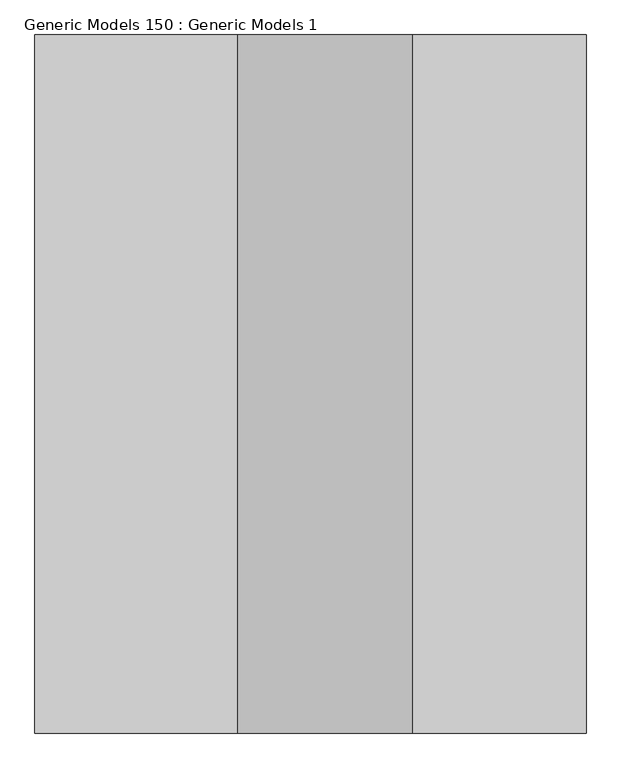
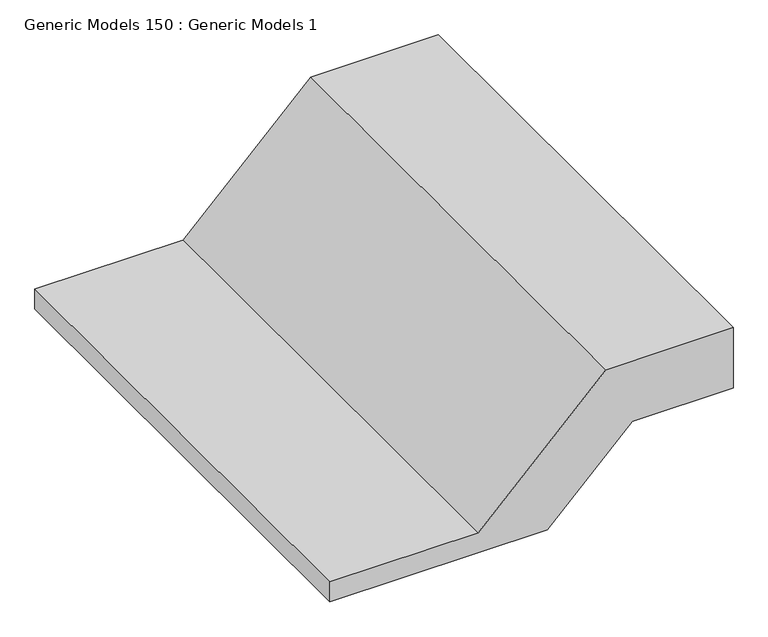
"""IFC4 building model written with IfcOpenShell, lengths in millimetres: proxy geometry, Generic Models 150 : Generic Models 1."""

import ifcopenshell
import ifcopenshell.guid

model = None  # the IFC model being written
_history = None  # IfcOwnerHistory: only IFC2X3 demands one
_inside = {}  # id of a spatial element -> (the spatial element, [elements in it])
_under = {}  # id of a project, library or spatial element -> (it, [spatial elements below it])
_declared = {}  # id of a project -> (the project, [libraries it declares])
_typed = {}  # id of a type object -> (the type object, [elements of that type])
_made_of = {}  # id of a material, layer set ... -> (it, [elements and type objects made of it])


def new_model(schema):
    """Start an empty IFC model of exactly this schema.

    Asked for "IFC4X3", IfcOpenShell would pick the latest addendum, in which some entities
    have other attributes; the version numbers below select the first issue.
    IFC2X3 requires an IfcOwnerHistory on every rooted entity: one is made here for all.
    """
    global model, _history
    if schema == "IFC4X3":
        model = ifcopenshell.file(schema_version=(4, 3, 0, 0))
    else:
        model = ifcopenshell.file(schema=schema)
    _inside.clear()
    _under.clear()
    _declared.clear()
    _typed.clear()
    _made_of.clear()
    _history = None
    if model.schema == "IFC2X3":
        org = make("IfcOrganization", Name="unknown")
        user = make(
            "IfcPersonAndOrganization",
            ThePerson=make("IfcPerson", FamilyName="unknown"),
            TheOrganization=org,
        )
        app = make(
            "IfcApplication",
            ApplicationDeveloper=org,
            Version="unknown",
            ApplicationFullName="unknown",
            ApplicationIdentifier="unknown",
        )
        _history = make(
            "IfcOwnerHistory",
            OwningUser=user,
            OwningApplication=app,
            ChangeAction="ADDED",
            CreationDate=0,
        )
    return model


def make(cls, **values):
    """One entity of the class cls with the attributes given. An attribute that is None is left unset."""
    return model.create_entity(
        cls, **{name: value for name, value in values.items() if value is not None}
    )


def rooted(cls, **values):
    """An entity with a GlobalId (a new one), such as an element, a storey or a relation."""
    return make(cls, GlobalId=ifcopenshell.guid.new(), OwnerHistory=_history, **values)


def si_unit(unit_type, name, prefix=None):
    """IfcSIUnit, for example si_unit("LENGTHUNIT", "METRE", prefix="MILLI")."""
    return make("IfcSIUnit", UnitType=unit_type, Prefix=prefix, Name=name)


def assignment(units):
    """IfcUnitAssignment: the units of a project."""
    return None if units is None else make("IfcUnitAssignment", Units=units)


def point(xyz):
    """IfcCartesianPoint."""
    return None if xyz is None else make("IfcCartesianPoint", Coordinates=xyz)


def direction(xyz):
    """IfcDirection."""
    return None if xyz is None else make("IfcDirection", DirectionRatios=xyz)


def frame(location, z_axis=None, x_axis=None):
    """IfcAxis2Placement3D, a coordinate frame: its origin and axes. An axis left out is left unset."""
    return make(
        "IfcAxis2Placement3D",
        Location=point(location),
        Axis=direction(z_axis),
        RefDirection=direction(x_axis),
    )


def origin():
    """The frame at (0, 0, 0) with its axes left unset."""
    return frame((0.0, 0.0, 0.0))


def place(relative_to, where):
    """IfcLocalPlacement: puts the frame where relative to a parent placement (None: the world)."""
    return make(
        "IfcLocalPlacement", PlacementRelTo=relative_to, RelativePlacement=where
    )


def context(
    kind, dimensions, precision=None, world=None, true_north=None, identifier=None
):
    """IfcGeometricRepresentationContext, for example the 3D "Model" context."""
    return make(
        "IfcGeometricRepresentationContext",
        ContextIdentifier=identifier,
        ContextType=kind,
        CoordinateSpaceDimension=dimensions,
        Precision=precision,
        WorldCoordinateSystem=world,
        TrueNorth=true_north,
    )


def project(units=None, contexts=None):
    """IfcProject with its units and contexts."""
    return rooted(
        "IfcProject",
        Name="project",
        RepresentationContexts=contexts,
        UnitsInContext=assignment(units),
    )


def spatial(cls, under=None, at=None, **own):
    """A site, building, storey or space (cls), placed at a placement, below another one or the project."""
    s = rooted(cls, ObjectPlacement=at, **own)
    if under is not None:
        _under.setdefault(under.id(), (under, []))[1].append(s)
    return s


def polyline(points):
    """IfcPolyline through the points."""
    return make("IfcPolyline", Points=[point(p) for p in points])


def outline(outer, holes=None, kind="AREA"):
    """IfcArbitraryClosedProfileDef: a profile drawn as a closed curve; with holes, ...WithVoids."""
    if holes is None:
        return make("IfcArbitraryClosedProfileDef", ProfileType=kind, OuterCurve=outer)
    return make(
        "IfcArbitraryProfileDefWithVoids",
        ProfileType=kind,
        OuterCurve=outer,
        InnerCurves=holes,
    )


def extrude(swept, where, along, depth):
    """IfcExtrudedAreaSolid: the profile swept, set in the frame where, extruded along a direction by depth."""
    return make(
        "IfcExtrudedAreaSolid",
        SweptArea=swept,
        Position=where,
        ExtrudedDirection=direction(along),
        Depth=depth,
    )


def shape(context_of_items, identifier, shape_type, items):
    """IfcShapeRepresentation: the items that make up one representation, for example the "Body"."""
    return make(
        "IfcShapeRepresentation",
        ContextOfItems=context_of_items,
        RepresentationIdentifier=identifier,
        RepresentationType=shape_type,
        Items=items,
    )


def source(mapping_origin, context_of_items, identifier, shape_type, items):
    """IfcRepresentationMap: a shape defined once, which mapped items show again and again."""
    return make(
        "IfcRepresentationMap",
        MappingOrigin=mapping_origin,
        MappedRepresentation=shape(context_of_items, identifier, shape_type, items),
    )


def transform(
    local_origin,
    x_axis=None,
    y_axis=None,
    z_axis=None,
    scale=None,
    scale2=None,
    scale3=None,
    uniform=True,
):
    """IfcCartesianTransformationOperator3D, or its non-uniform kind. x_axis, y_axis, z_axis: its Axis1, 2, 3."""
    if uniform:
        return make(
            "IfcCartesianTransformationOperator3D",
            Axis1=direction(x_axis),
            Axis2=direction(y_axis),
            LocalOrigin=point(local_origin),
            Scale=scale,
            Axis3=direction(z_axis),
        )
    return make(
        "IfcCartesianTransformationOperator3DnonUniform",
        Axis1=direction(x_axis),
        Axis2=direction(y_axis),
        LocalOrigin=point(local_origin),
        Scale=scale,
        Axis3=direction(z_axis),
        Scale2=scale2,
        Scale3=scale3,
    )


def mapped(mapping_source, mapping_target):
    """IfcMappedItem: shows the shape of a source again, moved by a transform."""
    return make(
        "IfcMappedItem", MappingSource=mapping_source, MappingTarget=mapping_target
    )


def made_of(thing, what):
    """Note that an element or type object is made of a material, layer set ...; save() writes the relation."""
    if what is not None:
        _made_of.setdefault(what.id(), (what, []))[1].append(thing)
    return thing


def element(
    cls,
    number,
    at=None,
    inside=None,
    cuts=None,
    type_object=None,
    material=None,
    context=None,
    identifier="Body",
    shape_type=None,
    held_by="IfcProductDefinitionShape",
    body=None,
    shapes=None,
    **own,
):
    """One element of the class cls, such as IfcWall. Its Tag is "e" and its number.

    at: its placement. inside: the storey or other place that contains it. cuts: it is an
    opening in that element (IfcRelVoidsElement). A single representation is given by context,
    identifier, shape_type and body (its items); several are given by shapes. held_by: the class
    of the entity that holds the representations. save() writes the other relations.
    """
    e = rooted(cls, Tag="e%d" % number, ObjectPlacement=at, **own)
    if body is not None:
        shapes = [shape(context, identifier, shape_type, body)]
    if shapes is not None:
        e.Representation = make(held_by, Representations=shapes)
    if inside is not None:
        _inside.setdefault(inside.id(), (inside, []))[1].append(e)
    if cuts is not None:
        rooted(
            "IfcRelVoidsElement", RelatingBuildingElement=cuts, RelatedOpeningElement=e
        )
    if type_object is not None:
        _typed.setdefault(type_object.id(), (type_object, []))[1].append(e)
    return made_of(e, material)


def aggregate(whole, parts):
    """IfcRelAggregates: a whole, such as a stair, and the parts it consists of."""
    return rooted("IfcRelAggregates", RelatingObject=whole, RelatedObjects=parts)


def save(model, path):
    """Write the relations noted so far, then the file.

    IfcRelAggregates (storeys below a building ...), IfcRelContainedInSpatialStructure (elements
    in a storey), IfcRelDefinesByType, IfcRelAssociatesMaterial and IfcRelDeclares: one each for
    every whole, place, type object, material and project.
    """
    for whole, parts in _under.values():
        aggregate(whole, parts)
    for where, things in _inside.values():
        rooted(
            "IfcRelContainedInSpatialStructure",
            RelatedElements=things,
            RelatingStructure=where,
        )
    for kind, things in _typed.values():
        rooted("IfcRelDefinesByType", RelatedObjects=things, RelatingType=kind)
    for what, things in _made_of.values():
        rooted("IfcRelAssociatesMaterial", RelatedObjects=things, RelatingMaterial=what)
    for by, libraries in _declared.values():
        rooted("IfcRelDeclares", RelatingContext=by, RelatedDefinitions=libraries)
    model.write(path)


def generic_models_150_generic_models_1_b2c8ea2b(model_context):
    return source(origin(), model_context, "Body", "SweptSolid", [
        extrude(outline(polyline([(-310.1710164, 52787.3395874), (-157.7710164, 52787.3395874), (-157.7710164, 52483.7302124), (-462.5710164, 52178.9302124), (-462.5710164, 51824.8420742), (-513.3710164, 51824.8420742), (-513.3710164, 52343.6563593), (-310.1710164, 52546.8563593), (-310.1710164, 52787.3395874)])), frame((0.0, 0.0, 0.0), z_axis=(0.0, 1.0, 0.0), x_axis=(0.0, 0.0, 1.0)), (0.0, 0.0, 1.0), 1219.2),
    ])


if __name__ == "__main__":
    model = new_model("IFC4")
    model_context = context("Model", 3, world=origin())
    ifc_project = project(units=[si_unit("LENGTHUNIT", "METRE", prefix="MILLI")], contexts=[model_context])
    site = spatial("IfcSite", under=ifc_project)
    building = spatial("IfcBuilding", under=site)
    placement = place(None, origin())
    generic_models_150_generic_models_1_shape = generic_models_150_generic_models_1_b2c8ea2b(model_context)
    element("IfcBuildingElementProxy", 1, Name="Generic Models 150 : Generic Models 1", ObjectType="Generic Models 150 : Generic Models 1", at=placement, inside=building, context=model_context, shape_type="MappedRepresentation", body=[
        mapped(generic_models_150_generic_models_1_shape, transform((0.0, 0.0, 0.0), x_axis=(1.0, 0.0, 0.0), y_axis=(0.0, 1.0, 0.0), z_axis=(0.0, 0.0, 1.0))),
    ])
    save(model, "model.ifc")

# Revit data of these elements
# Element 1 (IfcBuildingElementProxy, "Generic Models 150 : Generic Models 1")
#   Materials on its faces: "6\" COMPACTED CRUSHED STONE"
# Materials
#   "6\" COMPACTED CRUSHED STONE": class "Generic", colour RGB 255 255 255, transparency 0, Cost = 0
